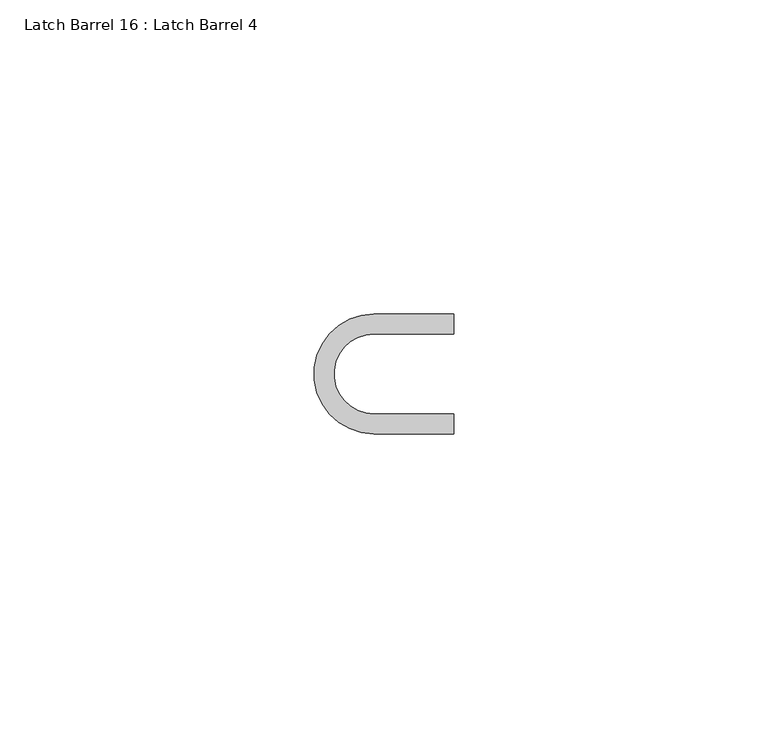
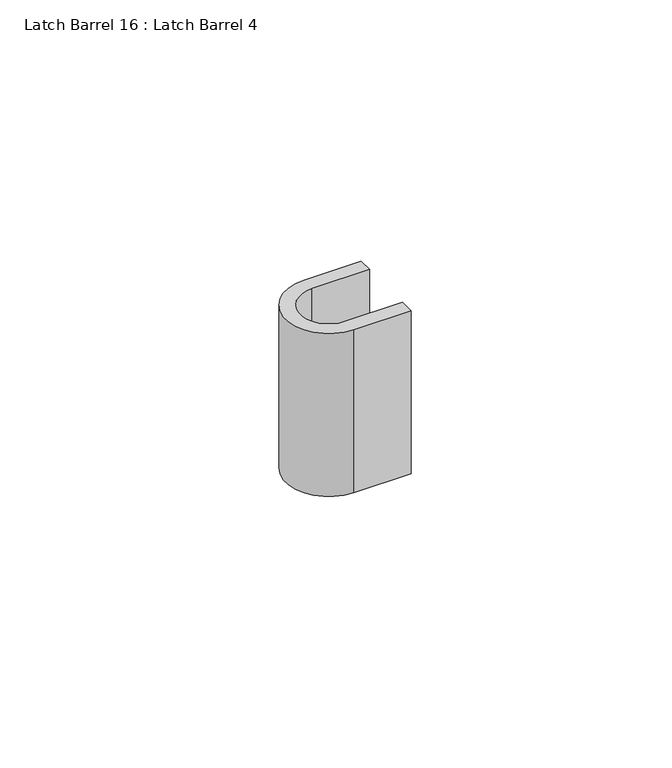
"""IFC4 building model written with IfcOpenShell, lengths in millimetres: proxy geometry, Latch Barrel 16 : Latch Barrel 4."""

from ifc_helpers import new_model, si_unit, point, frame, frame_2d, origin, place, context, project, spatial, polyline, circle_curve, trimmed, segment, composite_curve, outline, extrude, source, transform, mapped, element, save


def latch_barrel_16_latch_barrel_4_5b004ebd(model_context):
    return source(origin(), model_context, "Body", "SweptSolid", [
        extrude(outline(composite_curve([segment(trimmed(circle_curve(frame_2d((587309.5435739, -535163.4663841)), 6.35), [point((587309.5435739, -535157.1163841))], [point((587309.5435739, -535169.8163841))], True, "CARTESIAN"), True, "CONTINUOUS"), segment(polyline([(587309.5435739, -535169.8163841), (587322.2435739, -535169.8163841), (587322.2435739, -535172.9913841), (587309.5435739, -535172.9913841)]), True, "CONTINUOUS"), segment(trimmed(circle_curve(frame_2d((587309.5435739, -535163.4663841)), 9.525), [point((587309.5435739, -535172.9913841))], [point((587309.5435739, -535153.9413841))], False, "CARTESIAN"), True, "CONTINUOUS"), segment(polyline([(587309.5435739, -535153.9413841), (587322.2435739, -535153.9413841), (587322.2435739, -535157.1163841), (587309.5435739, -535157.1163841)]), True, "CONTINUOUS")], self_intersect=False)), frame((0.0, 0.0, 50.8), z_axis=(0.0, 0.0, 1.0), x_axis=(1.0, 0.0, 0.0)), (0.0, 0.0, 1.0), 38.1),
    ])


if __name__ == "__main__":
    model = new_model("IFC4")
    model_context = context("Model", 3, world=origin())
    ifc_project = project(units=[si_unit("LENGTHUNIT", "METRE", prefix="MILLI")], contexts=[model_context])
    site = spatial("IfcSite", under=ifc_project)
    building = spatial("IfcBuilding", under=site)
    placement = place(None, origin())
    latch_barrel_16_latch_barrel_4_shape = latch_barrel_16_latch_barrel_4_5b004ebd(model_context)
    element("IfcBuildingElementProxy", 1, Name="Latch Barrel 16 : Latch Barrel 4", ObjectType="Latch Barrel 16 : Latch Barrel 4", at=placement, inside=building, context=model_context, shape_type="MappedRepresentation", body=[
        mapped(latch_barrel_16_latch_barrel_4_shape, transform((0.0, 0.0, 0.0), x_axis=(1.0, 0.0, 0.0), y_axis=(0.0, 1.0, 0.0), z_axis=(0.0, 0.0, 1.0))),
    ])
    save(model, "model.ifc")

# Revit data of these elements
# Element 1 (IfcBuildingElementProxy, "Latch Barrel 16 : Latch Barrel 4")
#   Materials on its faces: "GALV. SLIDE BOLT"
# Materials
#   "GALV. SLIDE BOLT": class "Metal", colour RGB 189 187 185, transparency 0, Description = "Carbon steel", Cost = 0
